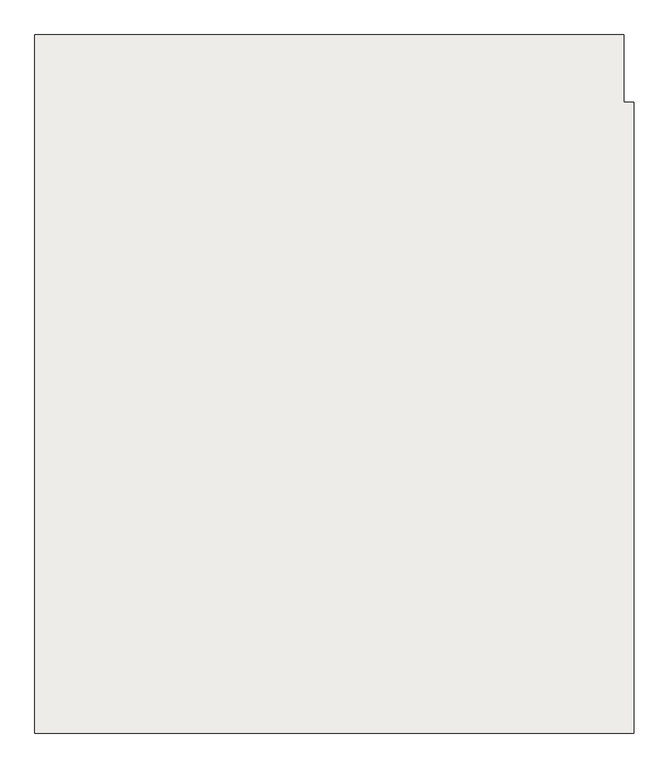
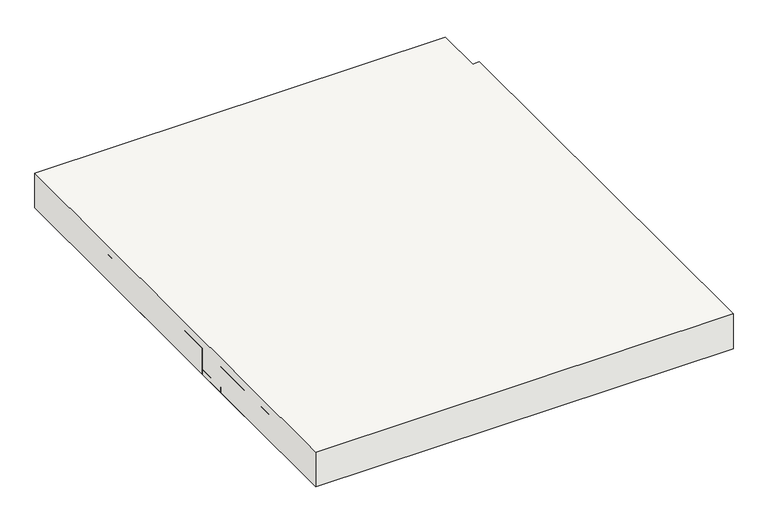
"""IFC4 building model written with IfcOpenShell, lengths in millimetres: slab geometry, Pano 11 (16 cm)."""

from ifc_helpers import new_model, si_unit, origin, origin_with_axes, place, context, project, spatial, polyline, outline, extrude, source, transform, mapped, element, save


def slab_ff925f6c(model_context):
    return source(origin(), model_context, "Body", "SweptSolid", [
        extrude(outline(polyline([(3940.0, 10355.0), (5730.0, 10355.0), (5730.0, 10150.0), (5760.0, 10150.0), (5760.0, 8235.0), (3940.0, 8235.0), (3940.0, 10355.0)])), origin_with_axes(), (0.0, 0.0, 1.0), 160.0),
        extrude(outline(polyline([(4940.0, 8590.0), (4940.0, 8950.0), (5435.0, 8950.0), (5435.0, 8590.0), (4940.0, 8590.0)])), origin_with_axes(), (0.0, 0.0, 1.0), 120.0),
        extrude(outline(polyline([(3940.0, 8450.0), (3940.0, 8590.0), (5760.0, 8590.0), (5760.0, 8450.0), (3940.0, 8450.0)])), origin_with_axes(), (0.0, 0.0, 1.0), 24.0),
        extrude(outline(polyline([(3940.0, 9090.0), (3940.0, 9450.0), (4435.0, 9450.0), (4435.0, 9090.0), (3940.0, 9090.0)])), origin_with_axes(), (0.0, 0.0, 1.0), 120.0),
        extrude(outline(polyline([(5440.0, 9090.0), (5440.0, 9450.0), (5755.0, 9450.0), (5755.0, 9090.0), (5440.0, 9090.0)])), origin_with_axes(), (0.0, 0.0, 1.0), 120.0),
        extrude(outline(polyline([(5440.0, 9590.0), (5440.0, 9950.0), (5755.0, 9950.0), (5755.0, 9590.0), (5440.0, 9590.0)])), origin_with_axes(), (0.0, 0.0, 1.0), 120.0),
        extrude(outline(polyline([(3940.0, 8590.0), (3940.0, 8950.0), (4435.0, 8950.0), (4435.0, 8590.0), (3940.0, 8590.0)])), origin_with_axes(), (0.0, 0.0, 1.0), 120.0),
        extrude(outline(polyline([(4940.0, 9090.0), (4940.0, 9450.0), (5435.0, 9450.0), (5435.0, 9090.0), (4940.0, 9090.0)])), origin_with_axes(), (0.0, 0.0, 1.0), 120.0),
        extrude(outline(polyline([(4940.0, 9590.0), (4940.0, 9950.0), (5435.0, 9950.0), (5435.0, 9590.0), (4940.0, 9590.0)])), origin_with_axes(), (0.0, 0.0, 1.0), 120.0),
        extrude(outline(polyline([(3940.0, 8950.0), (3940.0, 9090.0), (5760.0, 9090.0), (5760.0, 8950.0), (3940.0, 8950.0)])), origin_with_axes(), (0.0, 0.0, 1.0), 24.0),
        extrude(outline(polyline([(4440.0, 9590.0), (4440.0, 9950.0), (4935.0, 9950.0), (4935.0, 9590.0), (4440.0, 9590.0)])), origin_with_axes(), (0.0, 0.0, 1.0), 120.0),
        extrude(outline(polyline([(3940.0, 9450.0), (3940.0, 9590.0), (5760.0, 9590.0), (5760.0, 9450.0), (3940.0, 9450.0)])), origin_with_axes(), (0.0, 0.0, 1.0), 24.0),
        extrude(outline(polyline([(4440.0, 8590.0), (4440.0, 8950.0), (4935.0, 8950.0), (4935.0, 8590.0), (4440.0, 8590.0)])), origin_with_axes(), (0.0, 0.0, 1.0), 120.0),
        extrude(outline(polyline([(4440.0, 9090.0), (4440.0, 9450.0), (4935.0, 9450.0), (4935.0, 9090.0), (4440.0, 9090.0)])), origin_with_axes(), (0.0, 0.0, 1.0), 120.0),
        extrude(outline(polyline([(5440.0, 8590.0), (5440.0, 8950.0), (5755.0, 8950.0), (5755.0, 8590.0), (5440.0, 8590.0)])), origin_with_axes(), (0.0, 0.0, 1.0), 120.0),
        extrude(outline(polyline([(3940.0, 9950.0), (3940.0, 10090.0), (5760.0, 10090.0), (5760.0, 9950.0), (3940.0, 9950.0)])), origin_with_axes(), (0.0, 0.0, 1.0), 24.0),
        extrude(outline(polyline([(3940.0, 9590.0), (3940.0, 9950.0), (4435.0, 9950.0), (4435.0, 9590.0), (3940.0, 9590.0)])), origin_with_axes(), (0.0, 0.0, 1.0), 120.0),
    ])


if __name__ == "__main__":
    model = new_model("IFC4")
    model_context = context("Model", 3, world=origin())
    ifc_project = project(units=[si_unit("LENGTHUNIT", "METRE", prefix="MILLI")], contexts=[model_context])
    site = spatial("IfcSite", under=ifc_project)
    building = spatial("IfcBuilding", under=site)
    placement = place(None, origin())
    slab_shape = slab_ff925f6c(model_context)
    element("IfcSlab", 1, ObjectType="Pano 11 (16 cm)", at=placement, inside=building, context=model_context, shape_type="MappedRepresentation", body=[
        mapped(slab_shape, transform((0.0, 0.0, 0.0), x_axis=(1.0, 0.0, 0.0), y_axis=(0.0, 1.0, 0.0), z_axis=(0.0, 0.0, 1.0))),
    ])
    save(model, "model.ifc")

# Revit data of these elements
# Element 1 (IfcSlab, "Pano 11 (16 cm)")
#   Materials on its faces: "Molde de poliestireno", "Concreto armado", "RGB 168-169-158"
# Materials
#   "Molde de poliestireno": class "Não atribuído", colour RGB 255 255 255, transparency 0
#   "Concreto armado": class "Não atribuído", colour RGB 168 169 158, transparency 0
#   "RGB 168-169-158": class "Não atribuído", colour RGB 168 169 158, transparency 0
